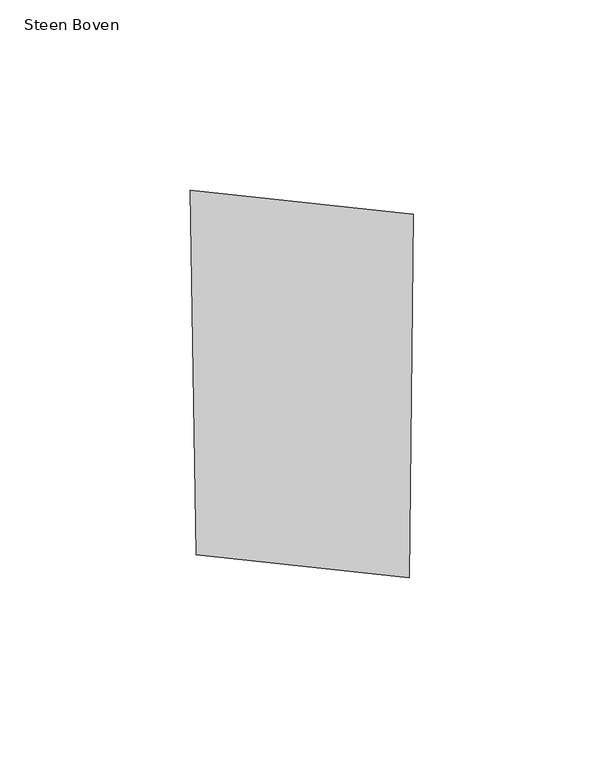
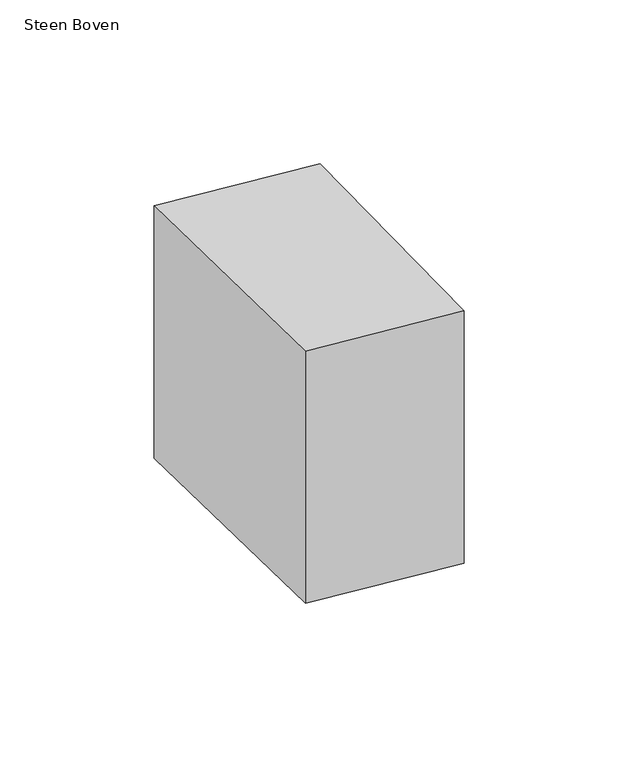
"""IFC4 building model written with IfcOpenShell, lengths in millimetres: proxy geometry, 00_GMA_steen_versie_4 : Steen Boven."""

from ifc_helpers import new_model, si_unit, origin, origin_with_axes, place, context, project, spatial, polyline, outline, extrude, source, transform, mapped, element, save


def steen_boven_0a1d95ac(model_context):
    return source(origin(), model_context, "Body", "SweptSolid", [
        extrude(outline(polyline([(101.1366322, 119.3612075), (100.0822343, 23.900879), (44.0625556, 29.9220432), (42.5102152, 125.6759088), (101.1366322, 119.3612075)])), origin_with_axes(), (0.0, 0.0, 1.0), 100.0),
    ])


if __name__ == "__main__":
    model = new_model("IFC4")
    model_context = context("Model", 3, world=origin())
    ifc_project = project(units=[si_unit("LENGTHUNIT", "METRE", prefix="MILLI")], contexts=[model_context])
    site = spatial("IfcSite", under=ifc_project)
    building = spatial("IfcBuilding", under=site)
    placement = place(None, origin())
    steen_boven_shape = steen_boven_0a1d95ac(model_context)
    element("IfcBuildingElementProxy", 1, Name="00_GMA_steen_versie_4 : Steen Boven", ObjectType="00_GMA_steen_versie_4 : Steen Boven", at=placement, inside=building, context=model_context, shape_type="MappedRepresentation", body=[
        mapped(steen_boven_shape, transform((0.0, 0.0, 0.0), x_axis=(1.0, 0.0, 0.0), y_axis=(0.0, 1.0, 0.0), z_axis=(0.0, 0.0, 1.0))),
    ])
    save(model, "model.ifc")

# Revit data of these elements
# Type "00_GMA_steen_versie_4 : Steen Boven"
#   StootVoegHalfBoven [instance default] = 5 mm
#   StootVoegHalf [instance default] = 5 mm
#   StootVoegBreedteOnder = 10 mm
#   StootVoegBreedteBoven = 10 mm
#   Steendikte = 100 mm
#   LintVoegOnderHalf = 5 mm
#   LintVoegOnder = 10 mm
#   LintVoegBovenHalf = 0 mm
#   LintVoegBoven = 0 mm
#   materiaal = none
#   MateriaalVoeg = none
#   Default Elevation = 0
